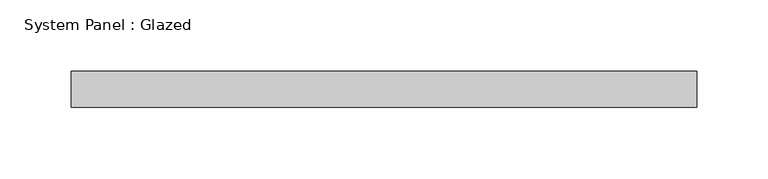
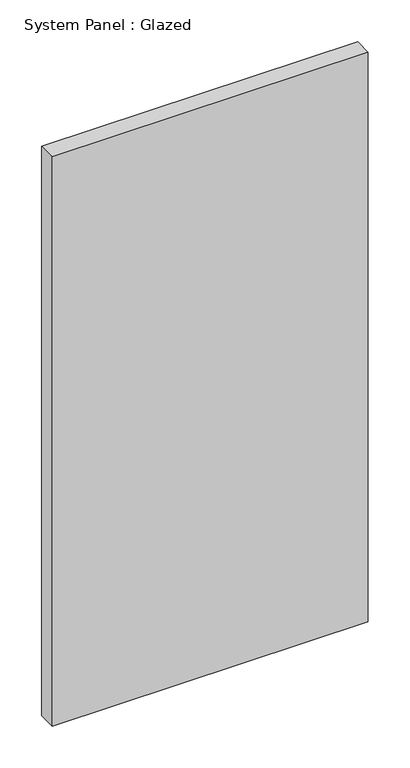
"""IFC4 building model written with IfcOpenShell, lengths in millimetres: plate geometry, System Panel : Glazed."""

from ifc_helpers import new_model, si_unit, origin, origin_with_axes, place, context, project, spatial, polyline, outline, extrude, source, transform, mapped, element, save


def system_panel_glazed_9f6fc0c4(model_context):
    return source(origin(), model_context, "Body", "SweptSolid", [
        extrude(outline(polyline([(218.9393939, 24.5), (-218.9393939, 24.5), (-218.9393939, 49.5), (218.9393939, 49.5), (218.9393939, 24.5)])), origin_with_axes(), (0.0, 0.0, 1.0), 833.3333333),
    ])


if __name__ == "__main__":
    model = new_model("IFC4")
    model_context = context("Model", 3, world=origin())
    ifc_project = project(units=[si_unit("LENGTHUNIT", "METRE", prefix="MILLI")], contexts=[model_context])
    site = spatial("IfcSite", under=ifc_project)
    building = spatial("IfcBuilding", under=site)
    placement = place(None, origin())
    system_panel_glazed_shape = system_panel_glazed_9f6fc0c4(model_context)
    element("IfcPlate", 1, ObjectType="System Panel : Glazed", at=placement, inside=building, context=model_context, shape_type="MappedRepresentation", body=[
        mapped(system_panel_glazed_shape, transform((0.0, 0.0, 0.0), x_axis=(1.0, 0.0, 0.0), y_axis=(0.0, 1.0, 0.0), z_axis=(0.0, 0.0, 1.0))),
    ])
    save(model, "model.ifc")

# Revit data of these elements
# Element 1 (IfcPlate, "System Panel : Glazed")
#   Materials on its faces: "Glass"
# Materials
#   "Glass": class "Glass", colour RGB 218 227 224, transparency 0.85, Description = "Soda Lime Glass", Cost = 0
